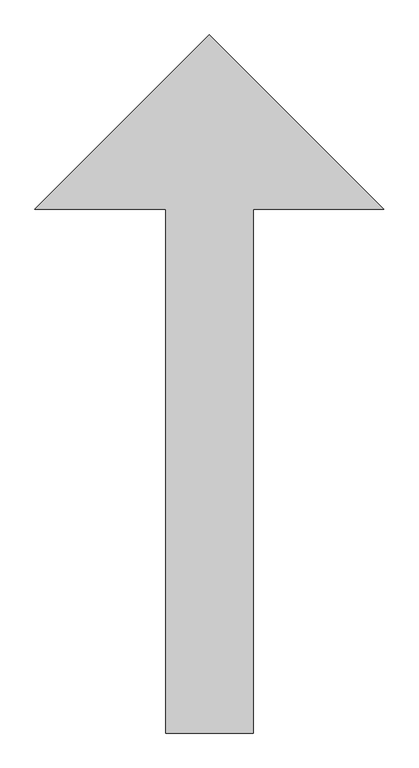
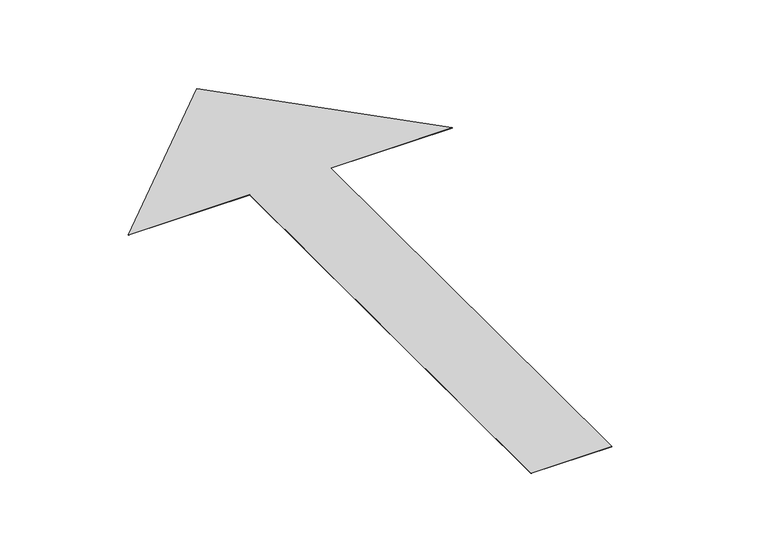
"""IFC4 building model written with IfcOpenShell, lengths in millimetres: proxy geometry, NLRS_90_PA_LB_pijl bewegwijzering_gen_rsf : pijl bewegwijzering."""

import ifcopenshell
import ifcopenshell.guid

model = None  # the IFC model being written
_history = None  # IfcOwnerHistory: only IFC2X3 demands one
_inside = {}  # id of a spatial element -> (the spatial element, [elements in it])
_under = {}  # id of a project, library or spatial element -> (it, [spatial elements below it])
_declared = {}  # id of a project -> (the project, [libraries it declares])
_typed = {}  # id of a type object -> (the type object, [elements of that type])
_made_of = {}  # id of a material, layer set ... -> (it, [elements and type objects made of it])


def new_model(schema):
    """Start an empty IFC model of exactly this schema.

    Asked for "IFC4X3", IfcOpenShell would pick the latest addendum, in which some entities
    have other attributes; the version numbers below select the first issue.
    IFC2X3 requires an IfcOwnerHistory on every rooted entity: one is made here for all.
    """
    global model, _history
    if schema == "IFC4X3":
        model = ifcopenshell.file(schema_version=(4, 3, 0, 0))
    else:
        model = ifcopenshell.file(schema=schema)
    _inside.clear()
    _under.clear()
    _declared.clear()
    _typed.clear()
    _made_of.clear()
    _history = None
    if model.schema == "IFC2X3":
        org = make("IfcOrganization", Name="unknown")
        user = make(
            "IfcPersonAndOrganization",
            ThePerson=make("IfcPerson", FamilyName="unknown"),
            TheOrganization=org,
        )
        app = make(
            "IfcApplication",
            ApplicationDeveloper=org,
            Version="unknown",
            ApplicationFullName="unknown",
            ApplicationIdentifier="unknown",
        )
        _history = make(
            "IfcOwnerHistory",
            OwningUser=user,
            OwningApplication=app,
            ChangeAction="ADDED",
            CreationDate=0,
        )
    return model


def make(cls, **values):
    """One entity of the class cls with the attributes given. An attribute that is None is left unset."""
    return model.create_entity(
        cls, **{name: value for name, value in values.items() if value is not None}
    )


def rooted(cls, **values):
    """An entity with a GlobalId (a new one), such as an element, a storey or a relation."""
    return make(cls, GlobalId=ifcopenshell.guid.new(), OwnerHistory=_history, **values)


def si_unit(unit_type, name, prefix=None):
    """IfcSIUnit, for example si_unit("LENGTHUNIT", "METRE", prefix="MILLI")."""
    return make("IfcSIUnit", UnitType=unit_type, Prefix=prefix, Name=name)


def assignment(units):
    """IfcUnitAssignment: the units of a project."""
    return None if units is None else make("IfcUnitAssignment", Units=units)


def point(xyz):
    """IfcCartesianPoint."""
    return None if xyz is None else make("IfcCartesianPoint", Coordinates=xyz)


def direction(xyz):
    """IfcDirection."""
    return None if xyz is None else make("IfcDirection", DirectionRatios=xyz)


def frame(location, z_axis=None, x_axis=None):
    """IfcAxis2Placement3D, a coordinate frame: its origin and axes. An axis left out is left unset."""
    return make(
        "IfcAxis2Placement3D",
        Location=point(location),
        Axis=direction(z_axis),
        RefDirection=direction(x_axis),
    )


def origin():
    """The frame at (0, 0, 0) with its axes left unset."""
    return frame((0.0, 0.0, 0.0))


def origin_with_axes():
    """The frame at (0, 0, 0) with the z axis (0, 0, 1) and the x axis (1, 0, 0) written out."""
    return frame((0.0, 0.0, 0.0), z_axis=(0.0, 0.0, 1.0), x_axis=(1.0, 0.0, 0.0))


def place(relative_to, where):
    """IfcLocalPlacement: puts the frame where relative to a parent placement (None: the world)."""
    return make(
        "IfcLocalPlacement", PlacementRelTo=relative_to, RelativePlacement=where
    )


def context(
    kind, dimensions, precision=None, world=None, true_north=None, identifier=None
):
    """IfcGeometricRepresentationContext, for example the 3D "Model" context."""
    return make(
        "IfcGeometricRepresentationContext",
        ContextIdentifier=identifier,
        ContextType=kind,
        CoordinateSpaceDimension=dimensions,
        Precision=precision,
        WorldCoordinateSystem=world,
        TrueNorth=true_north,
    )


def project(units=None, contexts=None):
    """IfcProject with its units and contexts."""
    return rooted(
        "IfcProject",
        Name="project",
        RepresentationContexts=contexts,
        UnitsInContext=assignment(units),
    )


def spatial(cls, under=None, at=None, **own):
    """A site, building, storey or space (cls), placed at a placement, below another one or the project."""
    s = rooted(cls, ObjectPlacement=at, **own)
    if under is not None:
        _under.setdefault(under.id(), (under, []))[1].append(s)
    return s


def polyline(points):
    """IfcPolyline through the points."""
    return make("IfcPolyline", Points=[point(p) for p in points])


def outline(outer, holes=None, kind="AREA"):
    """IfcArbitraryClosedProfileDef: a profile drawn as a closed curve; with holes, ...WithVoids."""
    if holes is None:
        return make("IfcArbitraryClosedProfileDef", ProfileType=kind, OuterCurve=outer)
    return make(
        "IfcArbitraryProfileDefWithVoids",
        ProfileType=kind,
        OuterCurve=outer,
        InnerCurves=holes,
    )


def extrude(swept, where, along, depth):
    """IfcExtrudedAreaSolid: the profile swept, set in the frame where, extruded along a direction by depth."""
    return make(
        "IfcExtrudedAreaSolid",
        SweptArea=swept,
        Position=where,
        ExtrudedDirection=direction(along),
        Depth=depth,
    )


def shape(context_of_items, identifier, shape_type, items):
    """IfcShapeRepresentation: the items that make up one representation, for example the "Body"."""
    return make(
        "IfcShapeRepresentation",
        ContextOfItems=context_of_items,
        RepresentationIdentifier=identifier,
        RepresentationType=shape_type,
        Items=items,
    )


def source(mapping_origin, context_of_items, identifier, shape_type, items):
    """IfcRepresentationMap: a shape defined once, which mapped items show again and again."""
    return make(
        "IfcRepresentationMap",
        MappingOrigin=mapping_origin,
        MappedRepresentation=shape(context_of_items, identifier, shape_type, items),
    )


def transform(
    local_origin,
    x_axis=None,
    y_axis=None,
    z_axis=None,
    scale=None,
    scale2=None,
    scale3=None,
    uniform=True,
):
    """IfcCartesianTransformationOperator3D, or its non-uniform kind. x_axis, y_axis, z_axis: its Axis1, 2, 3."""
    if uniform:
        return make(
            "IfcCartesianTransformationOperator3D",
            Axis1=direction(x_axis),
            Axis2=direction(y_axis),
            LocalOrigin=point(local_origin),
            Scale=scale,
            Axis3=direction(z_axis),
        )
    return make(
        "IfcCartesianTransformationOperator3DnonUniform",
        Axis1=direction(x_axis),
        Axis2=direction(y_axis),
        LocalOrigin=point(local_origin),
        Scale=scale,
        Axis3=direction(z_axis),
        Scale2=scale2,
        Scale3=scale3,
    )


def mapped(mapping_source, mapping_target):
    """IfcMappedItem: shows the shape of a source again, moved by a transform."""
    return make(
        "IfcMappedItem", MappingSource=mapping_source, MappingTarget=mapping_target
    )


def made_of(thing, what):
    """Note that an element or type object is made of a material, layer set ...; save() writes the relation."""
    if what is not None:
        _made_of.setdefault(what.id(), (what, []))[1].append(thing)
    return thing


def element(
    cls,
    number,
    at=None,
    inside=None,
    cuts=None,
    type_object=None,
    material=None,
    context=None,
    identifier="Body",
    shape_type=None,
    held_by="IfcProductDefinitionShape",
    body=None,
    shapes=None,
    **own,
):
    """One element of the class cls, such as IfcWall. Its Tag is "e" and its number.

    at: its placement. inside: the storey or other place that contains it. cuts: it is an
    opening in that element (IfcRelVoidsElement). A single representation is given by context,
    identifier, shape_type and body (its items); several are given by shapes. held_by: the class
    of the entity that holds the representations. save() writes the other relations.
    """
    e = rooted(cls, Tag="e%d" % number, ObjectPlacement=at, **own)
    if body is not None:
        shapes = [shape(context, identifier, shape_type, body)]
    if shapes is not None:
        e.Representation = make(held_by, Representations=shapes)
    if inside is not None:
        _inside.setdefault(inside.id(), (inside, []))[1].append(e)
    if cuts is not None:
        rooted(
            "IfcRelVoidsElement", RelatingBuildingElement=cuts, RelatedOpeningElement=e
        )
    if type_object is not None:
        _typed.setdefault(type_object.id(), (type_object, []))[1].append(e)
    return made_of(e, material)


def aggregate(whole, parts):
    """IfcRelAggregates: a whole, such as a stair, and the parts it consists of."""
    return rooted("IfcRelAggregates", RelatingObject=whole, RelatedObjects=parts)


def save(model, path):
    """Write the relations noted so far, then the file.

    IfcRelAggregates (storeys below a building ...), IfcRelContainedInSpatialStructure (elements
    in a storey), IfcRelDefinesByType, IfcRelAssociatesMaterial and IfcRelDeclares: one each for
    every whole, place, type object, material and project.
    """
    for whole, parts in _under.values():
        aggregate(whole, parts)
    for where, things in _inside.values():
        rooted(
            "IfcRelContainedInSpatialStructure",
            RelatedElements=things,
            RelatingStructure=where,
        )
    for kind, things in _typed.values():
        rooted("IfcRelDefinesByType", RelatedObjects=things, RelatingType=kind)
    for what, things in _made_of.values():
        rooted("IfcRelAssociatesMaterial", RelatedObjects=things, RelatingMaterial=what)
    for by, libraries in _declared.values():
        rooted("IfcRelDeclares", RelatingContext=by, RelatedDefinitions=libraries)
    model.write(path)


def parking_0bd23258(model_context):
    return source(origin(), model_context, "Body", "SweptSolid", [
        extrude(outline(polyline([(-125.0, 0.0), (375.0, -500.0), (0.0, -500.0), (0.0, -2000.0), (-250.0, -2000.0), (-250.0, -500.0), (-625.0, -500.0), (-125.0, 0.0)])), origin_with_axes(), (0.0, 0.0, 1.0), 1.0),
    ])


if __name__ == "__main__":
    model = new_model("IFC4")
    model_context = context("Model", 3, world=origin())
    ifc_project = project(units=[si_unit("LENGTHUNIT", "METRE", prefix="MILLI")], contexts=[model_context])
    site = spatial("IfcSite", under=ifc_project)
    building = spatial("IfcBuilding", under=site)
    placement = place(None, origin())
    parking_shape = parking_0bd23258(model_context)
    element("IfcBuildingElementProxy", 1, Name="NLRS_90_PA_LB_pijl bewegwijzering_gen_rsf : pijl bewegwijzering", ObjectType="NLRS_90_PA_LB_pijl bewegwijzering_gen_rsf : pijl bewegwijzering", at=placement, inside=building, context=model_context, shape_type="MappedRepresentation", body=[
        mapped(parking_shape, transform((0.0, 0.0, 0.0), x_axis=(1.0, 0.0, 0.0), y_axis=(0.0, 1.0, 0.0), z_axis=(0.0, 0.0, 1.0))),
    ])
    save(model, "model.ifc")

# Revit data of these elements
# Project information
#   Organization Name = "RSF"
#   Organization Description = "Revit Standards Foundation"
#   Building Name = "Onderwijsmodel Bouwkundig"
#   Author = "Emiel Ham TC-lid NLRS"
#   NLRS_C_opdrachtgever_adres = "Het Zuiderkruis 17, 5215 MV, 's-Hertogenbosch"
#   NLRS_C_opdrachtgever_contactpersoon = "Bestuur RSF"
#   NLRS_C_opdrachtgever_email = "secretary@revitstandards.org"
#   NLRS_C_opdrachtgever_projectnummer = "2017.4.015"
#   NLRS_C_opdrachtgever_telefoon = "nvt"
#   NLRS_C_project_email = "tc@revitstandards.org"
#   NLRS_C_project_kadaster_gemeente = "BIMSTAD"
#   NLRS_C_project_kadaster_nummer = "3"
#   NLRS_C_project_kadaster_sectie = "D"
#   NLRS_C_project_projectleider = "Martijn de Riet"
#   NLRS_C_project_telefoon = "+316 24 28 31 75"
#   NLRS_C_leverancier_bedrijfsnaam = "Technische Commissie RSF"
#   NLRS_C_leverancier_adres = "Het Zuiderkruis 17"
#   NLRS_C_leverancier_postcode = "5215 MV"
#   NLRS_C_leverancier_plaats = "'s-Hertogenbosch"
#   NLRS_C_leverancier_telefoonnummer = "nvt"
#   NLRS_C_leverancier_fax = "nvt"
#   NLRS_C_leverancier_email = "tc@revitstandards.org"
#   Workset = "Project Info"
#   IfcSite GUID = "3a0_Qb3mb9RuT4Z3SQBcsf"
#   IfcBuilding GUID = "3a0_Qb3mb9RuT4Z3SQBcsg"
#   IfcProject GUID = "3a0_Qb3mb9RuT4Z3SQBcsh"
#   Project Issue Date = "07-10-2021"
#   Project Status = "DEFINITIEF"
#   Client Name = "Revit Standards Foundation"
#   Project Address = "Onderwijsboulevard 123\n4567 HI Bimstad"
#   Project Name = "Onderwijsmodellen NLRS"
#   Project Number = "Onderwijsmodellen"
#   BCB_ProjectFolder = "C:\\Users\\Martijn de Riet\\Documents"
# Type "NLRS_90_PA_LB_pijl bewegwijzering_gen_rsf : pijl bewegwijzering"
#   Type IFC Predefined Type = "USERDEFINED"
#   Export Type to IFC As = "IfcBuildingElementProxyType"
#   Type IfcGUID = "2C9lkgojj1sel6c4s_vQ2Q"
#   IfcName[Type] = "pijl bewegwijzering"
#   IfcDescription[Type] = "pijl bewegwijzering"
#   IfcObjectType[Type] = "SIGNAGE"
#   Description = "pijl bewegwijzering"
#   Assembly Code = "90.72"
#   Pijlbreedte = 250.00 mm
#   Lengte_pijl = 2000.00 mm
#   Dikte_belijning = 1.00 mm
#   Materiaal_belijning = NLRS_v4_verf ivoorkleurig mat_gen_rsf
# Element 1 (IfcBuildingElementProxy, "NLRS_90_PA_LB_pijl bewegwijzering_gen_rsf : pijl bewegwijzering")
#   Materials on its faces: "NLRS_v4_verf ivoorkleurig mat_gen_rsf"
# Materials
#   "NLRS_v4_verf ivoorkleurig mat_gen_rsf": class "V - Verven", colour RGB 216 216 204, transparency 0, Keynote = "v4", Manufacturer = "Revit Standards Foundation", URL = "www.revitstandards.org", Description = "verf ivoorkleurig mat", Cost = 0
